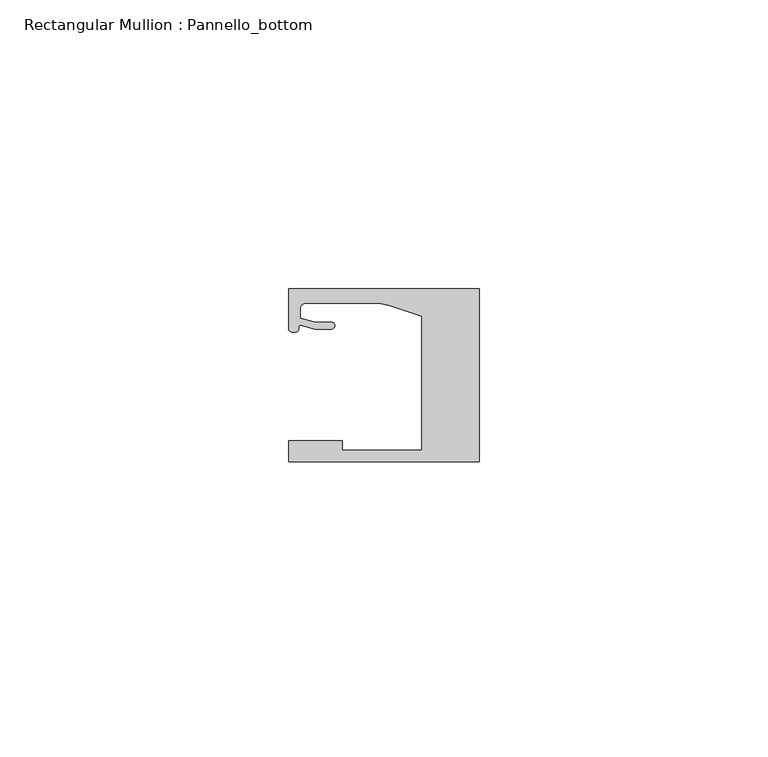
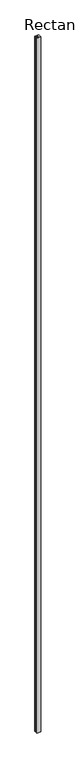
"""IFC4 building model written with IfcOpenShell, lengths in millimetres: member geometry, Rectangular Mullion : Pannello_bottom."""

import ifcopenshell
import ifcopenshell.guid

model = None  # the IFC model being written
_history = None  # IfcOwnerHistory: only IFC2X3 demands one
_inside = {}  # id of a spatial element -> (the spatial element, [elements in it])
_under = {}  # id of a project, library or spatial element -> (it, [spatial elements below it])
_declared = {}  # id of a project -> (the project, [libraries it declares])
_typed = {}  # id of a type object -> (the type object, [elements of that type])
_made_of = {}  # id of a material, layer set ... -> (it, [elements and type objects made of it])


def new_model(schema):
    """Start an empty IFC model of exactly this schema.

    Asked for "IFC4X3", IfcOpenShell would pick the latest addendum, in which some entities
    have other attributes; the version numbers below select the first issue.
    IFC2X3 requires an IfcOwnerHistory on every rooted entity: one is made here for all.
    """
    global model, _history
    if schema == "IFC4X3":
        model = ifcopenshell.file(schema_version=(4, 3, 0, 0))
    else:
        model = ifcopenshell.file(schema=schema)
    _inside.clear()
    _under.clear()
    _declared.clear()
    _typed.clear()
    _made_of.clear()
    _history = None
    if model.schema == "IFC2X3":
        org = make("IfcOrganization", Name="unknown")
        user = make(
            "IfcPersonAndOrganization",
            ThePerson=make("IfcPerson", FamilyName="unknown"),
            TheOrganization=org,
        )
        app = make(
            "IfcApplication",
            ApplicationDeveloper=org,
            Version="unknown",
            ApplicationFullName="unknown",
            ApplicationIdentifier="unknown",
        )
        _history = make(
            "IfcOwnerHistory",
            OwningUser=user,
            OwningApplication=app,
            ChangeAction="ADDED",
            CreationDate=0,
        )
    return model


def make(cls, **values):
    """One entity of the class cls with the attributes given. An attribute that is None is left unset."""
    return model.create_entity(
        cls, **{name: value for name, value in values.items() if value is not None}
    )


def rooted(cls, **values):
    """An entity with a GlobalId (a new one), such as an element, a storey or a relation."""
    return make(cls, GlobalId=ifcopenshell.guid.new(), OwnerHistory=_history, **values)


def si_unit(unit_type, name, prefix=None):
    """IfcSIUnit, for example si_unit("LENGTHUNIT", "METRE", prefix="MILLI")."""
    return make("IfcSIUnit", UnitType=unit_type, Prefix=prefix, Name=name)


def assignment(units):
    """IfcUnitAssignment: the units of a project."""
    return None if units is None else make("IfcUnitAssignment", Units=units)


def point(xyz):
    """IfcCartesianPoint."""
    return None if xyz is None else make("IfcCartesianPoint", Coordinates=xyz)


def direction(xyz):
    """IfcDirection."""
    return None if xyz is None else make("IfcDirection", DirectionRatios=xyz)


def frame(location, z_axis=None, x_axis=None):
    """IfcAxis2Placement3D, a coordinate frame: its origin and axes. An axis left out is left unset."""
    return make(
        "IfcAxis2Placement3D",
        Location=point(location),
        Axis=direction(z_axis),
        RefDirection=direction(x_axis),
    )


def origin():
    """The frame at (0, 0, 0) with its axes left unset."""
    return frame((0.0, 0.0, 0.0))


def place(relative_to, where):
    """IfcLocalPlacement: puts the frame where relative to a parent placement (None: the world)."""
    return make(
        "IfcLocalPlacement", PlacementRelTo=relative_to, RelativePlacement=where
    )


def context(
    kind, dimensions, precision=None, world=None, true_north=None, identifier=None
):
    """IfcGeometricRepresentationContext, for example the 3D "Model" context."""
    return make(
        "IfcGeometricRepresentationContext",
        ContextIdentifier=identifier,
        ContextType=kind,
        CoordinateSpaceDimension=dimensions,
        Precision=precision,
        WorldCoordinateSystem=world,
        TrueNorth=true_north,
    )


def project(units=None, contexts=None):
    """IfcProject with its units and contexts."""
    return rooted(
        "IfcProject",
        Name="project",
        RepresentationContexts=contexts,
        UnitsInContext=assignment(units),
    )


def spatial(cls, under=None, at=None, **own):
    """A site, building, storey or space (cls), placed at a placement, below another one or the project."""
    s = rooted(cls, ObjectPlacement=at, **own)
    if under is not None:
        _under.setdefault(under.id(), (under, []))[1].append(s)
    return s


def polyline(points):
    """IfcPolyline through the points."""
    return make("IfcPolyline", Points=[point(p) for p in points])


def circle_curve(where, radius):
    """IfcCircle in the frame where."""
    return make("IfcCircle", Position=where, Radius=radius)


def shape(context_of_items, identifier, shape_type, items):
    """IfcShapeRepresentation: the items that make up one representation, for example the "Body"."""
    return make(
        "IfcShapeRepresentation",
        ContextOfItems=context_of_items,
        RepresentationIdentifier=identifier,
        RepresentationType=shape_type,
        Items=items,
    )


def source(mapping_origin, context_of_items, identifier, shape_type, items):
    """IfcRepresentationMap: a shape defined once, which mapped items show again and again."""
    return make(
        "IfcRepresentationMap",
        MappingOrigin=mapping_origin,
        MappedRepresentation=shape(context_of_items, identifier, shape_type, items),
    )


def transform(
    local_origin,
    x_axis=None,
    y_axis=None,
    z_axis=None,
    scale=None,
    scale2=None,
    scale3=None,
    uniform=True,
):
    """IfcCartesianTransformationOperator3D, or its non-uniform kind. x_axis, y_axis, z_axis: its Axis1, 2, 3."""
    if uniform:
        return make(
            "IfcCartesianTransformationOperator3D",
            Axis1=direction(x_axis),
            Axis2=direction(y_axis),
            LocalOrigin=point(local_origin),
            Scale=scale,
            Axis3=direction(z_axis),
        )
    return make(
        "IfcCartesianTransformationOperator3DnonUniform",
        Axis1=direction(x_axis),
        Axis2=direction(y_axis),
        LocalOrigin=point(local_origin),
        Scale=scale,
        Axis3=direction(z_axis),
        Scale2=scale2,
        Scale3=scale3,
    )


def mapped(mapping_source, mapping_target):
    """IfcMappedItem: shows the shape of a source again, moved by a transform."""
    return make(
        "IfcMappedItem", MappingSource=mapping_source, MappingTarget=mapping_target
    )


def made_of(thing, what):
    """Note that an element or type object is made of a material, layer set ...; save() writes the relation."""
    if what is not None:
        _made_of.setdefault(what.id(), (what, []))[1].append(thing)
    return thing


def element(
    cls,
    number,
    at=None,
    inside=None,
    cuts=None,
    type_object=None,
    material=None,
    context=None,
    identifier="Body",
    shape_type=None,
    held_by="IfcProductDefinitionShape",
    body=None,
    shapes=None,
    **own,
):
    """One element of the class cls, such as IfcWall. Its Tag is "e" and its number.

    at: its placement. inside: the storey or other place that contains it. cuts: it is an
    opening in that element (IfcRelVoidsElement). A single representation is given by context,
    identifier, shape_type and body (its items); several are given by shapes. held_by: the class
    of the entity that holds the representations. save() writes the other relations.
    """
    e = rooted(cls, Tag="e%d" % number, ObjectPlacement=at, **own)
    if body is not None:
        shapes = [shape(context, identifier, shape_type, body)]
    if shapes is not None:
        e.Representation = make(held_by, Representations=shapes)
    if inside is not None:
        _inside.setdefault(inside.id(), (inside, []))[1].append(e)
    if cuts is not None:
        rooted(
            "IfcRelVoidsElement", RelatingBuildingElement=cuts, RelatedOpeningElement=e
        )
    if type_object is not None:
        _typed.setdefault(type_object.id(), (type_object, []))[1].append(e)
    return made_of(e, material)


def aggregate(whole, parts):
    """IfcRelAggregates: a whole, such as a stair, and the parts it consists of."""
    return rooted("IfcRelAggregates", RelatingObject=whole, RelatedObjects=parts)


def save(model, path):
    """Write the relations noted so far, then the file.

    IfcRelAggregates (storeys below a building ...), IfcRelContainedInSpatialStructure (elements
    in a storey), IfcRelDefinesByType, IfcRelAssociatesMaterial and IfcRelDeclares: one each for
    every whole, place, type object, material and project.
    """
    for whole, parts in _under.values():
        aggregate(whole, parts)
    for where, things in _inside.values():
        rooted(
            "IfcRelContainedInSpatialStructure",
            RelatedElements=things,
            RelatingStructure=where,
        )
    for kind, things in _typed.values():
        rooted("IfcRelDefinesByType", RelatedObjects=things, RelatingType=kind)
    for what, things in _made_of.values():
        rooted("IfcRelAssociatesMaterial", RelatedObjects=things, RelatingMaterial=what)
    for by, libraries in _declared.values():
        rooted("IfcRelDeclares", RelatingContext=by, RelatedDefinitions=libraries)
    model.write(path)


def plane_surface(at):
    """IfcPlane: the flat surface through the origin of the frame at, square to its z axis."""
    return make("IfcPlane", Position=at)


def cylinder_surface(at, radius):
    """IfcCylindricalSurface: all points at the distance radius from the z axis of the frame at."""
    return make("IfcCylindricalSurface", Position=at, Radius=radius)


def revolved_surface(curve, axis_point, axis_direction):
    """IfcSurfaceOfRevolution: the curve turned about the line through axis_point along axis_direction."""
    return make(
        "IfcSurfaceOfRevolution",
        SweptCurve=make("IfcArbitraryOpenProfileDef", ProfileType="CURVE", Curve=curve),
        AxisPosition=make("IfcAxis1Placement", Location=point(axis_point), Axis=direction(axis_direction)),
    )


def extruded_surface(curve, direction_of_extrusion, depth):
    """IfcSurfaceOfLinearExtrusion: the curve pushed along a direction by depth."""
    return make(
        "IfcSurfaceOfLinearExtrusion",
        SweptCurve=make("IfcArbitraryOpenProfileDef", ProfileType="CURVE", Curve=curve),
        ExtrudedDirection=direction(direction_of_extrusion),
        Depth=depth,
    )


def spline_curve(degree, points, multiplicities, knots, weights=None):
    """IfcBSplineCurveWithKnots; with weights, IfcRationalBSplineCurveWithKnots."""
    own = dict(
        Degree=degree,
        ControlPointsList=[point(p) for p in points],
        CurveForm="UNSPECIFIED",
        ClosedCurve=False,
        SelfIntersect=False,
        KnotMultiplicities=multiplicities,
        Knots=knots,
        KnotSpec="UNSPECIFIED",
    )
    if weights is None:
        return make("IfcBSplineCurveWithKnots", **own)
    return make("IfcRationalBSplineCurveWithKnots", WeightsData=weights, **own)


def advanced_brep(points, edges, surfaces, faces):
    """IfcAdvancedBrep: a solid bounded by faces that lie on surfaces and meet in shared edges.

    An edge is (start, end): straight between two places in points (the first is 0);
    or (start, end, curve); or (start, end, curve, False) where it runs against its curve.
    A face is (place in surfaces, loops), or (place, loops, False) where it looks against
    its surface's normal. A loop lists edges by number (the first is 1), with a minus sign
    where the edge is run from its end to its start. The first loop is the outer one.
    """
    corners = [point(p) for p in points]
    vertices = [make("IfcVertexPoint", VertexGeometry=c) for c in corners]
    made = []
    for start, end, *more in edges:
        made.append(
            make(
                "IfcEdgeCurve",
                EdgeStart=vertices[start],
                EdgeEnd=vertices[end],
                EdgeGeometry=more[0] if more else make("IfcPolyline", Points=[corners[start], corners[end]]),
                SameSense=more[1] if len(more) > 1 else True,
            )
        )
    hull = []
    for where, loops, *sense in faces:
        bounds = []
        for j, loop in enumerate(loops):
            ring = [make("IfcOrientedEdge", EdgeElement=made[abs(k) - 1], Orientation=k > 0) for k in loop]
            bounds.append(
                make(
                    "IfcFaceOuterBound" if j == 0 else "IfcFaceBound",
                    Bound=make("IfcEdgeLoop", EdgeList=ring),
                    Orientation=True,
                )
            )
        hull.append(make("IfcAdvancedFace", Bounds=bounds, FaceSurface=surfaces[where], SameSense=sense[0] if sense else True))
    return make("IfcAdvancedBrep", Outer=make("IfcClosedShell", CfsFaces=hull))


def rectangular_mullion_pannello_bottom_95d836da(model_context):
    return source(origin(), model_context, "Body", "AdvancedBrep", [
        advanced_brep(
        [(-33.0, -15.0, 0.0), (0.0, -15.0, 0.0), (0.0, 15.0, 0.0), (-33.0000135, 15.0, 0.0), (-33.0000135, 8.0000472, 0.0), (-30.9223017, 8.6490241, 0.0), (-28.4999305, 7.9999523, 0.0), (-25.59998, 7.9999523, 0.0), (-25.59998, 9.1999523, 0.0), (-28.3419477, 9.1999523, 0.0), (-31.0, 9.9121746, 0.0), (-31.0, 11.4999419, 0.0), (-30.0000002, 12.4999419, 0.0), (-18.5493024, 12.4999438, 0.0), (-15.4591336, 12.0105099, 0.0), (-9.9999723, 10.2367227, 0.0), (-9.9999723, -13.0000004, 0.0), (-23.700041, -13.0000004, 0.0), (-23.700041, -11.3000004, 0.0), (-33.0, -11.3000004, 0.0), (-33.0, -15.0, -6272.7890883), (-33.0, -11.3000004, -6272.7890883), (-23.700041, -11.3000004, -6272.7890883), (-23.700041, -13.0000004, -6272.7890883), (-9.9999723, -13.0000004, -6272.7890883), (-9.9999723, 10.2367227, -6272.7890883), (-15.4591336, 12.0105099, -6272.7890883), (-18.5493024, 12.4999438, -6272.7890883), (-30.0000002, 12.4999419, -6272.7890883), (-31.0, 11.4999419, -6272.7890883), (-31.0, 9.9121746, -6272.7890883), (-28.3419477, 9.1999523, -6272.7890883), (-25.59998, 9.1999523, -6272.7890883), (-25.59998, 7.9999523, -6272.7890883), (-28.4999305, 7.9999523, -6272.7890883), (-30.9223017, 8.6490241, -6272.7890883), (-33.0000135, 8.0000472, -6272.7890883), (-33.0000135, 15.0, -6272.7890883), (0.0, 15.0, -6272.7890883), (0.0, -15.0, -6272.7890883)],
        [
            (0, 1),
            (1, 2),
            (2, 3),
            (3, 4),
            (4, 5, spline_curve(3, [(-33.0000135, 8.0000472, 0.0), (-33.0000135, 7.457047519, 0.0), (-32.262327879, 7.456527435, 0.0), (-31.357433266, 7.563996614, 0.0), (-31.305645054, 7.690065204, 0.0), (-31.298563602, 8.366228555, 0.0), (-31.312054066, 8.717747958, 0.0), (-30.9223017, 8.6490241, 0.0)], [4, 2, 2, 4], [0.0, 0.0027053965905959043, 0.0058611956533709, 0.007702013405570312])),
            (5, 6),
            (6, 7),
            (7, 8, circle_curve(frame((-25.59998, 8.5999523, 0.0), z_axis=(0.0, 0.0, 1.0), x_axis=(0.0, 1.0, 0.0)), 0.6)),
            (8, 9),
            (9, 10),
            (10, 11),
            (11, 12, circle_curve(frame((-30.0, 11.4999419, 0.0), z_axis=(0.0, 0.0, -1.0), x_axis=(0.0, 1.0, 0.0)), 1.0)),
            (12, 13),
            (13, 14, circle_curve(frame((-18.5493007, 2.4999438, 0.0), z_axis=(0.0, 0.0, -1.0), x_axis=(0.0, 1.0, 0.0)), 10.0)),
            (14, 15),
            (15, 16),
            (16, 17),
            (17, 18),
            (18, 19),
            (19, 0),
            (20, 21),
            (21, 22),
            (22, 23),
            (23, 24),
            (24, 25),
            (25, 26),
            (26, 27, circle_curve(frame((-18.5493007, 2.4999438, -6272.7890883), z_axis=(0.0, 0.0, 1.0), x_axis=(0.0, 1.0, 0.0)), 10.0)),
            (27, 28),
            (28, 29, circle_curve(frame((-30.0, 11.4999419, -6272.7890883), z_axis=(0.0, 0.0, 1.0), x_axis=(0.0, 1.0, 0.0)), 1.0)),
            (29, 30),
            (30, 31),
            (31, 32),
            (32, 33, circle_curve(frame((-25.59998, 8.5999523, -6272.7890883), z_axis=(0.0, 0.0, -1.0), x_axis=(0.0, 1.0, 0.0)), 0.6)),
            (33, 34),
            (34, 35),
            (35, 36, spline_curve(3, [(-30.9223017, 8.6490241, -6272.7890883), (-31.312054066, 8.717747958, -6272.7890883), (-31.298563602, 8.366228555, -6272.7890883), (-31.305645054, 7.690065204, -6272.7890883), (-31.357433266, 7.563996614, -6272.7890883), (-32.262327879, 7.456527435, -6272.7890883), (-33.0000135, 7.457047519, -6272.7890883), (-33.0000135, 8.0000472, -6272.7890883)], [4, 2, 2, 4], [0.0, 0.001840817752199412, 0.004996616814974408, 0.007702013405570312])),
            (36, 37),
            (37, 38),
            (38, 39),
            (39, 20),
            (0, 20),
            (39, 1),
            (38, 2),
            (37, 3),
            (36, 4),
            (35, 5),
            (34, 6),
            (33, 7),
            (32, 8),
            (31, 9),
            (30, 10),
            (29, 11),
            (28, 12),
            (27, 13),
            (26, 14),
            (25, 15),
            (24, 16),
            (23, 17),
            (22, 18),
            (21, 19),
        ],
        [
            plane_surface(frame((0.0, -36.2491502, 0.0), z_axis=(0.0, 0.0, 1.0), x_axis=(-1.0, 0.0, 0.0))),
            plane_surface(frame((0.0, -36.2491502, -6272.7890883), z_axis=(0.0, 0.0, -1.0), x_axis=(-1.0, 0.0, 0.0))),
            plane_surface(frame((-33.0, -15.0, 0.0), z_axis=(0.0, -1.0, 0.0), x_axis=(0.0, 0.0, -1.0))),
            plane_surface(frame((0.0, -15.0, 0.0), z_axis=(1.0, 0.0, 0.0), x_axis=(0.0, 0.0, -1.0))),
            plane_surface(frame((0.0, 15.0, 0.0), z_axis=(0.0, 1.0, 0.0), x_axis=(0.0, 0.0, -1.0))),
            plane_surface(frame((-33.0000135, 15.0, 0.0), z_axis=(-1.0, 0.0, 0.0), x_axis=(0.0, 0.0, -1.0))),
            extruded_surface(spline_curve(3, [(-33.0000135, 8.0000472, -6272.7890883), (-33.0000135, 7.457047519, -6272.7890883), (-32.262327879, 7.456527435, -6272.7890883), (-31.357433266, 7.563996614, -6272.7890883), (-31.305645054, 7.690065204, -6272.7890883), (-31.298563602, 8.366228555, -6272.7890883), (-31.312054066, 8.717747958, -6272.7890883), (-30.9223017, 8.6490241, -6272.7890883)], [4, 2, 2, 4], [0.0, 0.0027053965905959043, 0.0058611956533709, 0.007702013405570312]), (0.0, 0.0, 6272.7890883), 6272.7890883),
            plane_surface(frame((-30.9223017, 8.6490241, 0.0), z_axis=(-0.25881883200192934, -0.9659258833891746, 0.0), x_axis=(0.0, 0.0, -1.0))),
            plane_surface(frame((-28.4999305, 7.9999523, 0.0), z_axis=(0.0, -1.0, 0.0), x_axis=(0.0, 0.0, -1.0))),
            cylinder_surface(frame((-25.59998, 8.5999523, 0.0), z_axis=(0.0, 0.0, 1.0), x_axis=(0.0, 1.0, 0.0)), 0.6),
            plane_surface(frame((-25.59998, 9.1999523, 0.0), z_axis=(0.0, 1.0, 0.0), x_axis=(0.0, 0.0, -1.0))),
            plane_surface(frame((-28.3419477, 9.1999523, 0.0), z_axis=(0.25881883204288636, 0.9659258833782002, 0.0), x_axis=(0.0, 0.0, -1.0))),
            plane_surface(frame((-31.0, 9.9121746, 0.0), z_axis=(1.0, 0.0, 0.0), x_axis=(0.0, 0.0, -1.0))),
            revolved_surface(polyline([(-30.0, 12.4999419, -6272.7890883), (-30.0, 12.4999419, 0.0)]), (-30.0, 11.4999419, 0.0), (0.0, 0.0, -1.0)),
            plane_surface(frame((-30.0000002, 12.4999419, 0.0), z_axis=(1.6923026533778639e-07, -0.9999999999999858, 0.0), x_axis=(0.0, 0.0, -1.0))),
            revolved_surface(polyline([(-18.5493007, 12.4999438, -6272.7890883), (-18.5493007, 12.4999438, 0.0)]), (-18.5493007, 2.4999438, 0.0), (0.0, 0.0, -1.0)),
            plane_surface(frame((-15.4591336, 12.0105099, 0.0), z_axis=(-0.30901670911956314, -0.9510566089801992, 0.0), x_axis=(0.0, 0.0, -1.0))),
            plane_surface(frame((-9.9999723, 10.2367227, 0.0), z_axis=(-1.0, 0.0, 0.0), x_axis=(0.0, 0.0, -1.0))),
            plane_surface(frame((-9.9999723, -13.0000004, 0.0), z_axis=(0.0, 1.0, 0.0), x_axis=(0.0, 0.0, -1.0))),
            plane_surface(frame((-23.700041, -13.0000004, 0.0), z_axis=(1.0, 0.0, 0.0), x_axis=(0.0, 0.0, -1.0))),
            plane_surface(frame((-23.700041, -11.3000004, 0.0), z_axis=(0.0, 1.0, 0.0), x_axis=(0.0, 0.0, -1.0))),
            plane_surface(frame((-33.0, -11.3000004, 0.0), z_axis=(-1.0, 0.0, 0.0), x_axis=(0.0, 0.0, -1.0))),
        ],
        [
            (0, [[1, 2, 3, 4, 5, 6, 7, 8, 9, 10, 11, 12, 13, 14, 15, 16, 17, 18, 19, 20]]),
            (1, [[21, 22, 23, 24, 25, 26, 27, 28, 29, 30, 31, 32, 33, 34, 35, 36, 37, 38, 39, 40]]),
            (2, [[-1, 41, -40, 42]]),
            (3, [[-2, -42, -39, 43]]),
            (4, [[-3, -43, -38, 44]]),
            (5, [[-4, -44, -37, 45]]),
            (6, [[-5, -45, -36, 46]]),
            (7, [[-6, -46, -35, 47]]),
            (8, [[-7, -47, -34, 48]]),
            (9, [[-8, -48, -33, 49]]),
            (10, [[-9, -49, -32, 50]]),
            (11, [[-10, -50, -31, 51]]),
            (12, [[-11, -51, -30, 52]]),
            (13, [[-12, -52, -29, 53]]),
            (14, [[-13, -53, -28, 54]]),
            (15, [[-14, -54, -27, 55]]),
            (16, [[-15, -55, -26, 56]]),
            (17, [[-16, -56, -25, 57]]),
            (18, [[-17, -57, -24, 58]]),
            (19, [[-18, -58, -23, 59]]),
            (20, [[-19, -59, -22, 60]]),
            (21, [[-20, -60, -21, -41]]),
        ],
    ),
    ])


if __name__ == "__main__":
    model = new_model("IFC4")
    model_context = context("Model", 3, world=origin())
    ifc_project = project(units=[si_unit("LENGTHUNIT", "METRE", prefix="MILLI")], contexts=[model_context])
    site = spatial("IfcSite", under=ifc_project)
    building = spatial("IfcBuilding", under=site)
    placement = place(None, origin())
    rectangular_mullion_pannello_bottom_shape = rectangular_mullion_pannello_bottom_95d836da(model_context)
    element("IfcMember", 1, ObjectType="Rectangular Mullion : Pannello_bottom", at=placement, inside=building, context=model_context, shape_type="MappedRepresentation", body=[
        mapped(rectangular_mullion_pannello_bottom_shape, transform((0.0, 0.0, 0.0), x_axis=(1.0, 0.0, 0.0), y_axis=(0.0, 1.0, 0.0), z_axis=(0.0, 0.0, 1.0))),
    ])
    save(model, "model.ifc")

# Revit data of these elements
# Type "Rectangular Mullion : Pannello_bottom"
#   built-in parameter 1007322 = 0.0984252 (stored number, unit not read)
#   built-in parameter 1007321 = 0.0328083 (stored number, unit not read)
#   built-in parameter 1007320 = 0 (stored number, unit not read)
